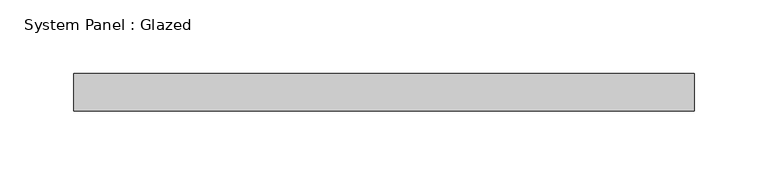
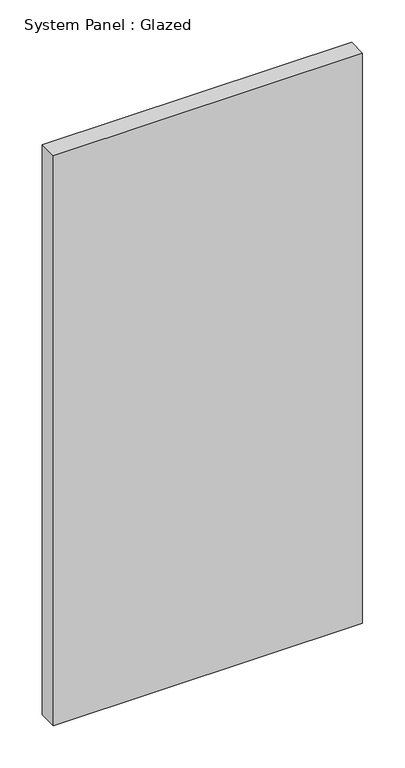
"""IFC4 building model written with IfcOpenShell, lengths in millimetres: plate geometry, System Panel : Glazed."""

from ifc_helpers import new_model, si_unit, origin, origin_with_axes, place, context, project, spatial, polyline, outline, extrude, source, transform, mapped, element, save


def system_panel_glazed_0b46a978(model_context):
    return source(origin(), model_context, "Body", "SweptSolid", [
        extrude(outline(polyline([(210.1070235, 19.05), (-210.1070235, 19.05), (-210.1070235, 44.45), (210.1070235, 44.45), (210.1070235, 19.05)])), origin_with_axes(), (0.0, 0.0, 1.0), 819.15),
    ])


if __name__ == "__main__":
    model = new_model("IFC4")
    model_context = context("Model", 3, world=origin())
    ifc_project = project(units=[si_unit("LENGTHUNIT", "METRE", prefix="MILLI")], contexts=[model_context])
    site = spatial("IfcSite", under=ifc_project)
    building = spatial("IfcBuilding", under=site)
    placement = place(None, origin())
    system_panel_glazed_shape = system_panel_glazed_0b46a978(model_context)
    element("IfcPlate", 1, ObjectType="System Panel : Glazed", at=placement, inside=building, context=model_context, shape_type="MappedRepresentation", body=[
        mapped(system_panel_glazed_shape, transform((0.0, 0.0, 0.0), x_axis=(1.0, 0.0, 0.0), y_axis=(0.0, 1.0, 0.0), z_axis=(0.0, 0.0, 1.0))),
    ])
    save(model, "model.ifc")

# Revit data of these elements
# Element 1 (IfcPlate, "System Panel : Glazed")
#   Materials on its faces: "Glass"
# Materials
#   "Glass": class "Glass", colour RGB 0 128 192, transparency 0.75
